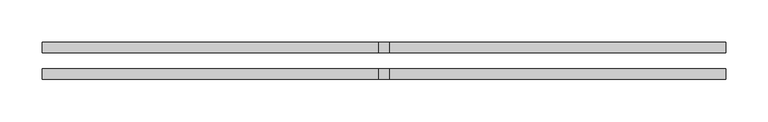
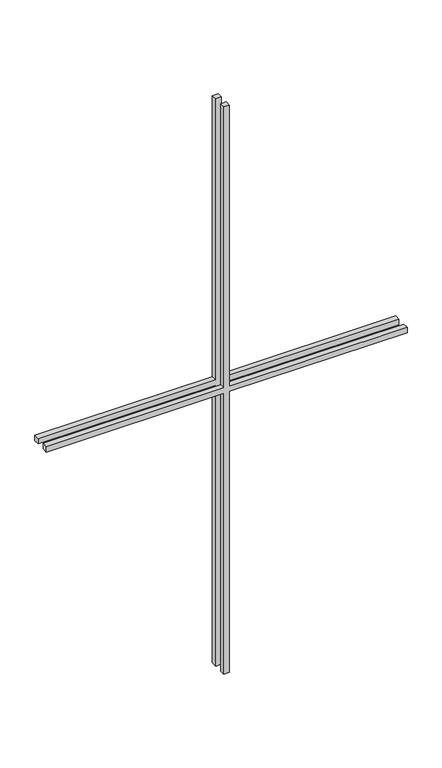
"""IFC4 building model written with IfcOpenShell, lengths in millimetres: proxy geometry, M_Padrão do montante_2x2 : M_Padrão do montante_2x2."""

import ifcopenshell
import ifcopenshell.guid

model = None  # the IFC model being written
_history = None  # IfcOwnerHistory: only IFC2X3 demands one
_inside = {}  # id of a spatial element -> (the spatial element, [elements in it])
_under = {}  # id of a project, library or spatial element -> (it, [spatial elements below it])
_declared = {}  # id of a project -> (the project, [libraries it declares])
_typed = {}  # id of a type object -> (the type object, [elements of that type])
_made_of = {}  # id of a material, layer set ... -> (it, [elements and type objects made of it])


def new_model(schema):
    """Start an empty IFC model of exactly this schema.

    Asked for "IFC4X3", IfcOpenShell would pick the latest addendum, in which some entities
    have other attributes; the version numbers below select the first issue.
    IFC2X3 requires an IfcOwnerHistory on every rooted entity: one is made here for all.
    """
    global model, _history
    if schema == "IFC4X3":
        model = ifcopenshell.file(schema_version=(4, 3, 0, 0))
    else:
        model = ifcopenshell.file(schema=schema)
    _inside.clear()
    _under.clear()
    _declared.clear()
    _typed.clear()
    _made_of.clear()
    _history = None
    if model.schema == "IFC2X3":
        org = make("IfcOrganization", Name="unknown")
        user = make(
            "IfcPersonAndOrganization",
            ThePerson=make("IfcPerson", FamilyName="unknown"),
            TheOrganization=org,
        )
        app = make(
            "IfcApplication",
            ApplicationDeveloper=org,
            Version="unknown",
            ApplicationFullName="unknown",
            ApplicationIdentifier="unknown",
        )
        _history = make(
            "IfcOwnerHistory",
            OwningUser=user,
            OwningApplication=app,
            ChangeAction="ADDED",
            CreationDate=0,
        )
    return model


def make(cls, **values):
    """One entity of the class cls with the attributes given. An attribute that is None is left unset."""
    return model.create_entity(
        cls, **{name: value for name, value in values.items() if value is not None}
    )


def rooted(cls, **values):
    """An entity with a GlobalId (a new one), such as an element, a storey or a relation."""
    return make(cls, GlobalId=ifcopenshell.guid.new(), OwnerHistory=_history, **values)


def si_unit(unit_type, name, prefix=None):
    """IfcSIUnit, for example si_unit("LENGTHUNIT", "METRE", prefix="MILLI")."""
    return make("IfcSIUnit", UnitType=unit_type, Prefix=prefix, Name=name)


def assignment(units):
    """IfcUnitAssignment: the units of a project."""
    return None if units is None else make("IfcUnitAssignment", Units=units)


def point(xyz):
    """IfcCartesianPoint."""
    return None if xyz is None else make("IfcCartesianPoint", Coordinates=xyz)


def direction(xyz):
    """IfcDirection."""
    return None if xyz is None else make("IfcDirection", DirectionRatios=xyz)


def frame(location, z_axis=None, x_axis=None):
    """IfcAxis2Placement3D, a coordinate frame: its origin and axes. An axis left out is left unset."""
    return make(
        "IfcAxis2Placement3D",
        Location=point(location),
        Axis=direction(z_axis),
        RefDirection=direction(x_axis),
    )


def origin():
    """The frame at (0, 0, 0) with its axes left unset."""
    return frame((0.0, 0.0, 0.0))


def place(relative_to, where):
    """IfcLocalPlacement: puts the frame where relative to a parent placement (None: the world)."""
    return make(
        "IfcLocalPlacement", PlacementRelTo=relative_to, RelativePlacement=where
    )


def context(
    kind, dimensions, precision=None, world=None, true_north=None, identifier=None
):
    """IfcGeometricRepresentationContext, for example the 3D "Model" context."""
    return make(
        "IfcGeometricRepresentationContext",
        ContextIdentifier=identifier,
        ContextType=kind,
        CoordinateSpaceDimension=dimensions,
        Precision=precision,
        WorldCoordinateSystem=world,
        TrueNorth=true_north,
    )


def project(units=None, contexts=None):
    """IfcProject with its units and contexts."""
    return rooted(
        "IfcProject",
        Name="project",
        RepresentationContexts=contexts,
        UnitsInContext=assignment(units),
    )


def spatial(cls, under=None, at=None, **own):
    """A site, building, storey or space (cls), placed at a placement, below another one or the project."""
    s = rooted(cls, ObjectPlacement=at, **own)
    if under is not None:
        _under.setdefault(under.id(), (under, []))[1].append(s)
    return s


def polyline(points):
    """IfcPolyline through the points."""
    return make("IfcPolyline", Points=[point(p) for p in points])


def outline(outer, holes=None, kind="AREA"):
    """IfcArbitraryClosedProfileDef: a profile drawn as a closed curve; with holes, ...WithVoids."""
    if holes is None:
        return make("IfcArbitraryClosedProfileDef", ProfileType=kind, OuterCurve=outer)
    return make(
        "IfcArbitraryProfileDefWithVoids",
        ProfileType=kind,
        OuterCurve=outer,
        InnerCurves=holes,
    )


def extrude(swept, where, along, depth):
    """IfcExtrudedAreaSolid: the profile swept, set in the frame where, extruded along a direction by depth."""
    return make(
        "IfcExtrudedAreaSolid",
        SweptArea=swept,
        Position=where,
        ExtrudedDirection=direction(along),
        Depth=depth,
    )


def shape(context_of_items, identifier, shape_type, items):
    """IfcShapeRepresentation: the items that make up one representation, for example the "Body"."""
    return make(
        "IfcShapeRepresentation",
        ContextOfItems=context_of_items,
        RepresentationIdentifier=identifier,
        RepresentationType=shape_type,
        Items=items,
    )


def source(mapping_origin, context_of_items, identifier, shape_type, items):
    """IfcRepresentationMap: a shape defined once, which mapped items show again and again."""
    return make(
        "IfcRepresentationMap",
        MappingOrigin=mapping_origin,
        MappedRepresentation=shape(context_of_items, identifier, shape_type, items),
    )


def transform(
    local_origin,
    x_axis=None,
    y_axis=None,
    z_axis=None,
    scale=None,
    scale2=None,
    scale3=None,
    uniform=True,
):
    """IfcCartesianTransformationOperator3D, or its non-uniform kind. x_axis, y_axis, z_axis: its Axis1, 2, 3."""
    if uniform:
        return make(
            "IfcCartesianTransformationOperator3D",
            Axis1=direction(x_axis),
            Axis2=direction(y_axis),
            LocalOrigin=point(local_origin),
            Scale=scale,
            Axis3=direction(z_axis),
        )
    return make(
        "IfcCartesianTransformationOperator3DnonUniform",
        Axis1=direction(x_axis),
        Axis2=direction(y_axis),
        LocalOrigin=point(local_origin),
        Scale=scale,
        Axis3=direction(z_axis),
        Scale2=scale2,
        Scale3=scale3,
    )


def mapped(mapping_source, mapping_target):
    """IfcMappedItem: shows the shape of a source again, moved by a transform."""
    return make(
        "IfcMappedItem", MappingSource=mapping_source, MappingTarget=mapping_target
    )


def made_of(thing, what):
    """Note that an element or type object is made of a material, layer set ...; save() writes the relation."""
    if what is not None:
        _made_of.setdefault(what.id(), (what, []))[1].append(thing)
    return thing


def element(
    cls,
    number,
    at=None,
    inside=None,
    cuts=None,
    type_object=None,
    material=None,
    context=None,
    identifier="Body",
    shape_type=None,
    held_by="IfcProductDefinitionShape",
    body=None,
    shapes=None,
    **own,
):
    """One element of the class cls, such as IfcWall. Its Tag is "e" and its number.

    at: its placement. inside: the storey or other place that contains it. cuts: it is an
    opening in that element (IfcRelVoidsElement). A single representation is given by context,
    identifier, shape_type and body (its items); several are given by shapes. held_by: the class
    of the entity that holds the representations. save() writes the other relations.
    """
    e = rooted(cls, Tag="e%d" % number, ObjectPlacement=at, **own)
    if body is not None:
        shapes = [shape(context, identifier, shape_type, body)]
    if shapes is not None:
        e.Representation = make(held_by, Representations=shapes)
    if inside is not None:
        _inside.setdefault(inside.id(), (inside, []))[1].append(e)
    if cuts is not None:
        rooted(
            "IfcRelVoidsElement", RelatingBuildingElement=cuts, RelatedOpeningElement=e
        )
    if type_object is not None:
        _typed.setdefault(type_object.id(), (type_object, []))[1].append(e)
    return made_of(e, material)


def aggregate(whole, parts):
    """IfcRelAggregates: a whole, such as a stair, and the parts it consists of."""
    return rooted("IfcRelAggregates", RelatingObject=whole, RelatedObjects=parts)


def save(model, path):
    """Write the relations noted so far, then the file.

    IfcRelAggregates (storeys below a building ...), IfcRelContainedInSpatialStructure (elements
    in a storey), IfcRelDefinesByType, IfcRelAssociatesMaterial and IfcRelDeclares: one each for
    every whole, place, type object, material and project.
    """
    for whole, parts in _under.values():
        aggregate(whole, parts)
    for where, things in _inside.values():
        rooted(
            "IfcRelContainedInSpatialStructure",
            RelatedElements=things,
            RelatingStructure=where,
        )
    for kind, things in _typed.values():
        rooted("IfcRelDefinesByType", RelatedObjects=things, RelatingType=kind)
    for what, things in _made_of.values():
        rooted("IfcRelAssociatesMaterial", RelatedObjects=things, RelatingMaterial=what)
    for by, libraries in _declared.values():
        rooted("IfcRelDeclares", RelatingContext=by, RelatedDefinitions=libraries)
    model.write(path)


def generic_models_3ff90e20(model_context):
    return source(origin(), model_context, "Body", "SweptSolid", [
        extrude(outline(polyline([(683.325, -6.35), (683.325, -407.1375), (670.625, -407.1375), (670.625, -6.35), (0.0, -6.35), (0.0, 6.35), (670.625, 6.35), (670.625, 407.1375), (683.325, 407.1375), (683.325, 6.35), (1353.95, 6.35), (1353.95, -6.35), (683.325, -6.35)])), frame((0.0, 9.525, 0.0), z_axis=(0.0, 1.0, 0.0), x_axis=(0.0, 0.0, 1.0)), (0.0, 0.0, 1.0), 12.7),
        extrude(outline(polyline([(683.325, -6.35), (683.325, -407.1375), (670.625, -407.1375), (670.625, -6.35), (0.0, -6.35), (0.0, 6.35), (670.625, 6.35), (670.625, 407.1375), (683.325, 407.1375), (683.325, 6.35), (1353.95, 6.35), (1353.95, -6.35), (683.325, -6.35)])), frame((0.0, -22.225, 0.0), z_axis=(0.0, 1.0, 0.0), x_axis=(0.0, 0.0, 1.0)), (0.0, 0.0, 1.0), 12.7),
    ])


if __name__ == "__main__":
    model = new_model("IFC4")
    model_context = context("Model", 3, world=origin())
    ifc_project = project(units=[si_unit("LENGTHUNIT", "METRE", prefix="MILLI")], contexts=[model_context])
    site = spatial("IfcSite", under=ifc_project)
    building = spatial("IfcBuilding", under=site)
    placement = place(None, origin())
    generic_models_shape = generic_models_3ff90e20(model_context)
    element("IfcBuildingElementProxy", 1, Name="M_Padrão do montante_2x2 : M_Padrão do montante_2x2", ObjectType="M_Padrão do montante_2x2 : M_Padrão do montante_2x2", at=placement, inside=building, context=model_context, shape_type="MappedRepresentation", body=[
        mapped(generic_models_shape, transform((0.0, 0.0, 0.0), x_axis=(1.0, 0.0, 0.0), y_axis=(0.0, 1.0, 0.0), z_axis=(0.0, 0.0, 1.0))),
    ])
    save(model, "model.ifc")

# Revit data of these elements
# Project information
#   Nome da organização = "FFR"
#   Autor = "Fernando"
#   MCI_ProjInf_tipo_de_projeto = "Residêncial"
#   Data de emissão do projeto = "Data de emissão"
#   Status do projeto = "Status do projeto"
#   Nome do cliente = "Proprietário"
#   Endereço do projeto = "Insira aqui o endereço"
#   Nome do projeto = "Projeto exemplo MIC"
#   Número do projeto = "A001"
# Type "M_Padrão do montante_2x2 : M_Padrão do montante_2x2"
#   Largura [instance default] = 1.200 m
#   Espessura = 0.0127 m
#   Altura [instance default] = 1.200 m
#   Distância = 0.01905 m
#   Material interior [instance default] = none
#   Material externo [instance default] = none
#   Default Elevation = 0
# Element 1 (IfcBuildingElementProxy, "M_Padrão do montante_2x2 : M_Padrão do montante_2x2")
#   Largura = 0.814275 m
#   Altura = 1.35395 m
#   Material interior = Madeira – Manchada
#   Material externo = Revestimento – Branco
#   Materials on its faces: "Revestimento – Branco", "Madeira – Manchada"
# Materials
#   "Revestimento – Branco": class "Madeira", colour RGB 242 242 238, transparency 0, Cost = 0
#   "Madeira – Manchada": class "Madeira", colour RGB 224 178 126, transparency 0, Cost = 0
